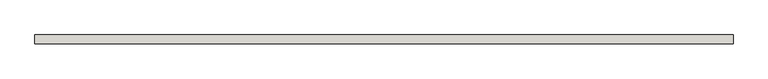
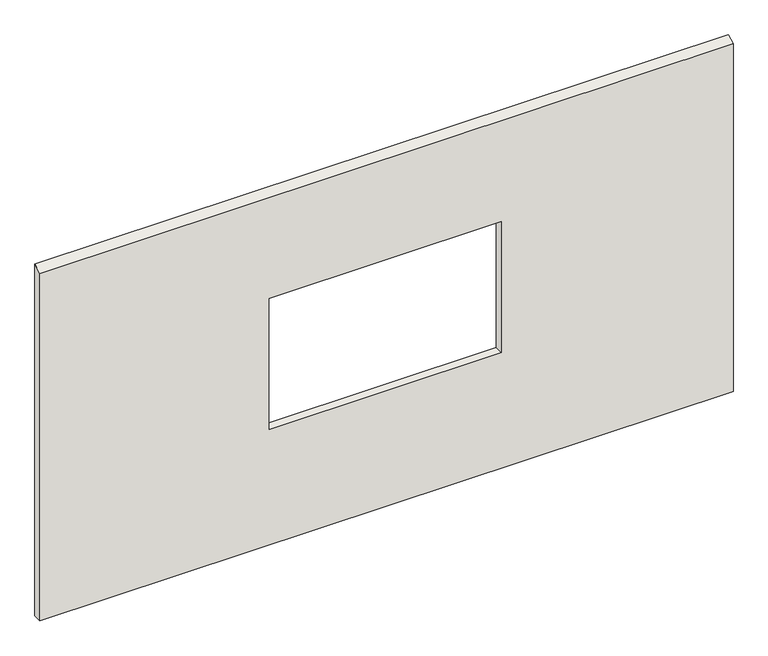
"""IFC4 building model written with IfcOpenShell, lengths in millimetres: wall geometry, 0_3d."""

from ifc_helpers import new_model, si_unit, origin, place, context, project, spatial, faceted_brep, source, transform, mapped, element, save


def wall_22845782(model_context):
    return source(origin(), model_context, "Body", "Brep", [
        faceted_brep([(1875.0, 70.0, 1000.0), (1875.0, 70.0, 2135.0), (1875.0, 0.0, 2135.0), (1875.0, 0.0, 1000.0), (3775.0, 70.0, 2135.0), (3775.0, 0.0, 2135.0), (3775.0, 70.0, 1000.0), (3775.0, 0.0, 1000.0), (0.0, 0.0, 3007.913011), (5670.0, 0.0, 3007.913011), (5670.0, 70.0, 3043.5797924), (0.0, 70.0, 3043.5797924), (5670.0, 0.0, 0.0), (5670.0, 70.0, 0.0), (0.0, 0.0, 0.0), (0.0, 70.0, 0.0)], [[[0, 1, 2, 3]], [[1, 4, 5, 2]], [[4, 6, 7, 5]], [[6, 0, 3, 7]], [[8, 9, 10, 11]], [[10, 9, 12, 13]], [[9, 8, 14, 12], [3, 2, 5, 7]], [[8, 11, 15, 14]], [[13, 15, 11, 10], [1, 0, 6, 4]], [[13, 12, 14, 15]]]),
    ])


if __name__ == "__main__":
    model = new_model("IFC4")
    model_context = context("Model", 3, world=origin())
    ifc_project = project(units=[si_unit("LENGTHUNIT", "METRE", prefix="MILLI")], contexts=[model_context])
    site = spatial("IfcSite", under=ifc_project)
    building = spatial("IfcBuilding", under=site)
    placement = place(None, origin())
    wall_shape = wall_22845782(model_context)
    element("IfcWall", 1, ObjectType="0_3d", at=placement, inside=building, context=model_context, shape_type="MappedRepresentation", body=[
        mapped(wall_shape, transform((0.0, 0.0, 0.0), x_axis=(1.0, 0.0, 0.0), y_axis=(0.0, 1.0, 0.0), z_axis=(0.0, 0.0, 1.0))),
    ])
    save(model, "model.ifc")

# Revit data of these elements
# Element 1 (IfcWall, "0_3d")
#   Materials on its faces: "Glass_Simple"
# Materials
#   "Glass_Simple": class "Unassigned", colour RGB 255 255 255, transparency 0.9
